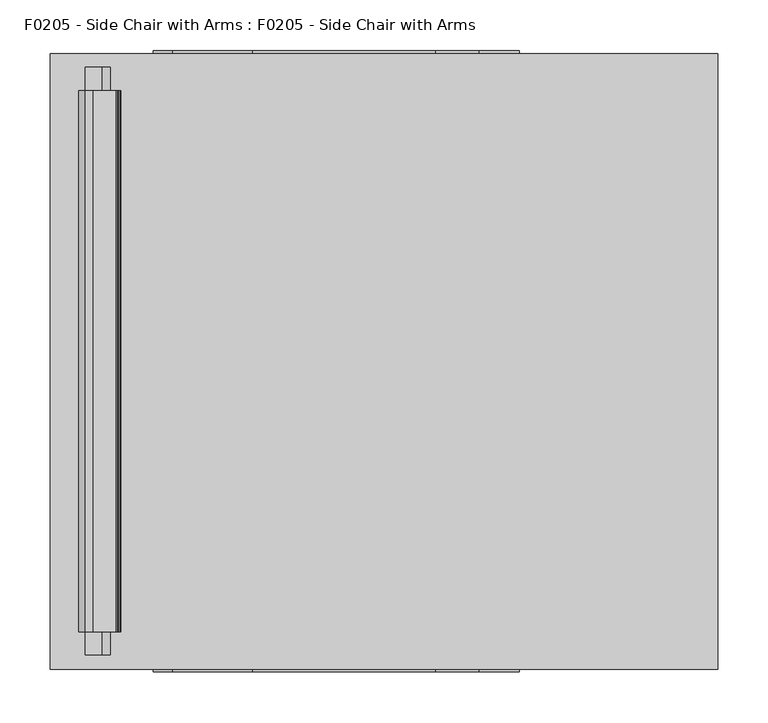
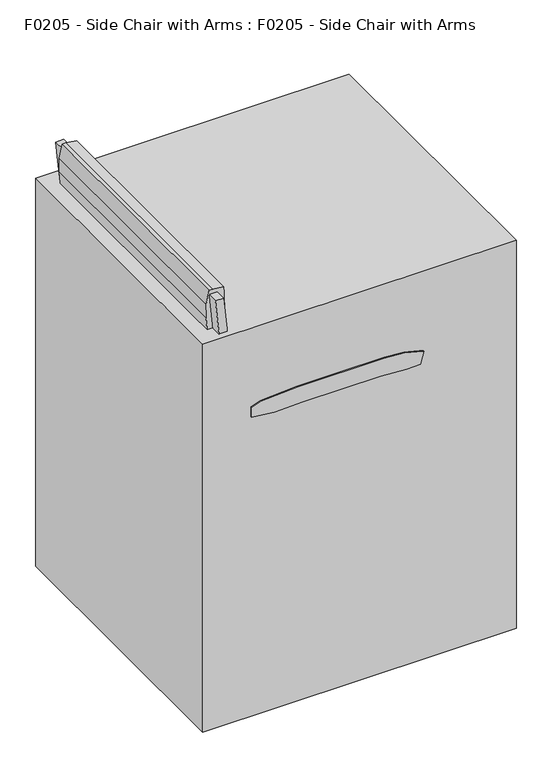
"""IFC4 building model written with IfcOpenShell, lengths in millimetres: proxy geometry, F0205 - Side Chair with Arms : F0205 - Side Chair with Arms."""

import ifcopenshell
import ifcopenshell.guid

model = None  # the IFC model being written
_history = None  # IfcOwnerHistory: only IFC2X3 demands one
_inside = {}  # id of a spatial element -> (the spatial element, [elements in it])
_under = {}  # id of a project, library or spatial element -> (it, [spatial elements below it])
_declared = {}  # id of a project -> (the project, [libraries it declares])
_typed = {}  # id of a type object -> (the type object, [elements of that type])
_made_of = {}  # id of a material, layer set ... -> (it, [elements and type objects made of it])


def new_model(schema):
    """Start an empty IFC model of exactly this schema.

    Asked for "IFC4X3", IfcOpenShell would pick the latest addendum, in which some entities
    have other attributes; the version numbers below select the first issue.
    IFC2X3 requires an IfcOwnerHistory on every rooted entity: one is made here for all.
    """
    global model, _history
    if schema == "IFC4X3":
        model = ifcopenshell.file(schema_version=(4, 3, 0, 0))
    else:
        model = ifcopenshell.file(schema=schema)
    _inside.clear()
    _under.clear()
    _declared.clear()
    _typed.clear()
    _made_of.clear()
    _history = None
    if model.schema == "IFC2X3":
        org = make("IfcOrganization", Name="unknown")
        user = make(
            "IfcPersonAndOrganization",
            ThePerson=make("IfcPerson", FamilyName="unknown"),
            TheOrganization=org,
        )
        app = make(
            "IfcApplication",
            ApplicationDeveloper=org,
            Version="unknown",
            ApplicationFullName="unknown",
            ApplicationIdentifier="unknown",
        )
        _history = make(
            "IfcOwnerHistory",
            OwningUser=user,
            OwningApplication=app,
            ChangeAction="ADDED",
            CreationDate=0,
        )
    return model


def make(cls, **values):
    """One entity of the class cls with the attributes given. An attribute that is None is left unset."""
    return model.create_entity(
        cls, **{name: value for name, value in values.items() if value is not None}
    )


def rooted(cls, **values):
    """An entity with a GlobalId (a new one), such as an element, a storey or a relation."""
    return make(cls, GlobalId=ifcopenshell.guid.new(), OwnerHistory=_history, **values)


def si_unit(unit_type, name, prefix=None):
    """IfcSIUnit, for example si_unit("LENGTHUNIT", "METRE", prefix="MILLI")."""
    return make("IfcSIUnit", UnitType=unit_type, Prefix=prefix, Name=name)


def assignment(units):
    """IfcUnitAssignment: the units of a project."""
    return None if units is None else make("IfcUnitAssignment", Units=units)


def point(xyz):
    """IfcCartesianPoint."""
    return None if xyz is None else make("IfcCartesianPoint", Coordinates=xyz)


def direction(xyz):
    """IfcDirection."""
    return None if xyz is None else make("IfcDirection", DirectionRatios=xyz)


def frame(location, z_axis=None, x_axis=None):
    """IfcAxis2Placement3D, a coordinate frame: its origin and axes. An axis left out is left unset."""
    return make(
        "IfcAxis2Placement3D",
        Location=point(location),
        Axis=direction(z_axis),
        RefDirection=direction(x_axis),
    )


def origin():
    """The frame at (0, 0, 0) with its axes left unset."""
    return frame((0.0, 0.0, 0.0))


def origin_with_axes():
    """The frame at (0, 0, 0) with the z axis (0, 0, 1) and the x axis (1, 0, 0) written out."""
    return frame((0.0, 0.0, 0.0), z_axis=(0.0, 0.0, 1.0), x_axis=(1.0, 0.0, 0.0))


def place(relative_to, where):
    """IfcLocalPlacement: puts the frame where relative to a parent placement (None: the world)."""
    return make(
        "IfcLocalPlacement", PlacementRelTo=relative_to, RelativePlacement=where
    )


def context(
    kind, dimensions, precision=None, world=None, true_north=None, identifier=None
):
    """IfcGeometricRepresentationContext, for example the 3D "Model" context."""
    return make(
        "IfcGeometricRepresentationContext",
        ContextIdentifier=identifier,
        ContextType=kind,
        CoordinateSpaceDimension=dimensions,
        Precision=precision,
        WorldCoordinateSystem=world,
        TrueNorth=true_north,
    )


def project(units=None, contexts=None):
    """IfcProject with its units and contexts."""
    return rooted(
        "IfcProject",
        Name="project",
        RepresentationContexts=contexts,
        UnitsInContext=assignment(units),
    )


def spatial(cls, under=None, at=None, **own):
    """A site, building, storey or space (cls), placed at a placement, below another one or the project."""
    s = rooted(cls, ObjectPlacement=at, **own)
    if under is not None:
        _under.setdefault(under.id(), (under, []))[1].append(s)
    return s


def polyline(points):
    """IfcPolyline through the points."""
    return make("IfcPolyline", Points=[point(p) for p in points])


def outline(outer, holes=None, kind="AREA"):
    """IfcArbitraryClosedProfileDef: a profile drawn as a closed curve; with holes, ...WithVoids."""
    if holes is None:
        return make("IfcArbitraryClosedProfileDef", ProfileType=kind, OuterCurve=outer)
    return make(
        "IfcArbitraryProfileDefWithVoids",
        ProfileType=kind,
        OuterCurve=outer,
        InnerCurves=holes,
    )


def extrude(swept, where, along, depth):
    """IfcExtrudedAreaSolid: the profile swept, set in the frame where, extruded along a direction by depth."""
    return make(
        "IfcExtrudedAreaSolid",
        SweptArea=swept,
        Position=where,
        ExtrudedDirection=direction(along),
        Depth=depth,
    )


def shape(context_of_items, identifier, shape_type, items):
    """IfcShapeRepresentation: the items that make up one representation, for example the "Body"."""
    return make(
        "IfcShapeRepresentation",
        ContextOfItems=context_of_items,
        RepresentationIdentifier=identifier,
        RepresentationType=shape_type,
        Items=items,
    )


def source(mapping_origin, context_of_items, identifier, shape_type, items):
    """IfcRepresentationMap: a shape defined once, which mapped items show again and again."""
    return make(
        "IfcRepresentationMap",
        MappingOrigin=mapping_origin,
        MappedRepresentation=shape(context_of_items, identifier, shape_type, items),
    )


def transform(
    local_origin,
    x_axis=None,
    y_axis=None,
    z_axis=None,
    scale=None,
    scale2=None,
    scale3=None,
    uniform=True,
):
    """IfcCartesianTransformationOperator3D, or its non-uniform kind. x_axis, y_axis, z_axis: its Axis1, 2, 3."""
    if uniform:
        return make(
            "IfcCartesianTransformationOperator3D",
            Axis1=direction(x_axis),
            Axis2=direction(y_axis),
            LocalOrigin=point(local_origin),
            Scale=scale,
            Axis3=direction(z_axis),
        )
    return make(
        "IfcCartesianTransformationOperator3DnonUniform",
        Axis1=direction(x_axis),
        Axis2=direction(y_axis),
        LocalOrigin=point(local_origin),
        Scale=scale,
        Axis3=direction(z_axis),
        Scale2=scale2,
        Scale3=scale3,
    )


def mapped(mapping_source, mapping_target):
    """IfcMappedItem: shows the shape of a source again, moved by a transform."""
    return make(
        "IfcMappedItem", MappingSource=mapping_source, MappingTarget=mapping_target
    )


def made_of(thing, what):
    """Note that an element or type object is made of a material, layer set ...; save() writes the relation."""
    if what is not None:
        _made_of.setdefault(what.id(), (what, []))[1].append(thing)
    return thing


def element(
    cls,
    number,
    at=None,
    inside=None,
    cuts=None,
    type_object=None,
    material=None,
    context=None,
    identifier="Body",
    shape_type=None,
    held_by="IfcProductDefinitionShape",
    body=None,
    shapes=None,
    **own,
):
    """One element of the class cls, such as IfcWall. Its Tag is "e" and its number.

    at: its placement. inside: the storey or other place that contains it. cuts: it is an
    opening in that element (IfcRelVoidsElement). A single representation is given by context,
    identifier, shape_type and body (its items); several are given by shapes. held_by: the class
    of the entity that holds the representations. save() writes the other relations.
    """
    e = rooted(cls, Tag="e%d" % number, ObjectPlacement=at, **own)
    if body is not None:
        shapes = [shape(context, identifier, shape_type, body)]
    if shapes is not None:
        e.Representation = make(held_by, Representations=shapes)
    if inside is not None:
        _inside.setdefault(inside.id(), (inside, []))[1].append(e)
    if cuts is not None:
        rooted(
            "IfcRelVoidsElement", RelatingBuildingElement=cuts, RelatedOpeningElement=e
        )
    if type_object is not None:
        _typed.setdefault(type_object.id(), (type_object, []))[1].append(e)
    return made_of(e, material)


def aggregate(whole, parts):
    """IfcRelAggregates: a whole, such as a stair, and the parts it consists of."""
    return rooted("IfcRelAggregates", RelatingObject=whole, RelatedObjects=parts)


def save(model, path):
    """Write the relations noted so far, then the file.

    IfcRelAggregates (storeys below a building ...), IfcRelContainedInSpatialStructure (elements
    in a storey), IfcRelDefinesByType, IfcRelAssociatesMaterial and IfcRelDeclares: one each for
    every whole, place, type object, material and project.
    """
    for whole, parts in _under.values():
        aggregate(whole, parts)
    for where, things in _inside.values():
        rooted(
            "IfcRelContainedInSpatialStructure",
            RelatedElements=things,
            RelatingStructure=where,
        )
    for kind, things in _typed.values():
        rooted("IfcRelDefinesByType", RelatedObjects=things, RelatingType=kind)
    for what, things in _made_of.values():
        rooted("IfcRelAssociatesMaterial", RelatedObjects=things, RelatingMaterial=what)
    for by, libraries in _declared.values():
        rooted("IfcRelDeclares", RelatingContext=by, RelatedDefinitions=libraries)
    model.write(path)


def f0205_side_chair_with_arms_f0205_side_chair_with_arms_598bf5c1(model_context):
    return source(origin(), model_context, "Body", "SweptSolid", [
        extrude(outline(polyline([(949.5558695, -288.1891828), (949.0276678, -295.7428189), (920.9464532, -302.0388283), (890.9596762, -302.364601), (766.4444592, -291.4709311), (712.0444312, -282.2922915), (699.4048634, -275.0755148), (701.6800869, -249.0695909), (734.5347731, -247.5019251), (744.2301544, -248.5209507), (775.1826091, -252.8120869), (831.1136295, -257.7054171), (872.5802588, -261.3332771), (887.0899422, -262.6027099), (935.3234911, -264.152458), (946.525946, -265.1325458), (949.5558695, -288.1891828)])), frame((0.0, -267.8488342, 0.0), z_axis=(0.0, 1.0, 0.0), x_axis=(0.0, 0.0, 1.0)), (0.0, 0.0, 1.0), 536.2041409),
        extrude(outline(polyline([(-256.4009052, 523.5214117), (-241.6696752, 524.0358376), (0.2532363, 511.5153378), (242.1729901, 524.0426254), (256.8914817, 523.5286444), (268.3553067, 472.7447876), (248.2006555, 466.9655344), (0.2531025, 454.1861401), (-247.7015659, 466.8926254), (-267.8488342, 472.7447876), (-256.4009052, 523.5214117)])), frame((-276.0175852, 0.0, 0.0), z_axis=(1.0, 0.0, 0.0), x_axis=(0.0, 1.0, 0.0)), (0.0, 0.0, 1.0), 448.6997704),
        extrude(outline(polyline([(688.7736743, -228.6), (667.1445431, -228.6), (661.9341602, -181.3714246), (664.006805, -120.3965081), (664.006805, 42.1384065), (660.8978378, 96.9044584), (660.8978378, 126.6899316), (687.4154537, 134.0660802), (697.5043243, 94.4420938), (700.8875965, 51.2519248), (700.8875965, -129.7992697), (695.7892437, -209.3248816), (688.7736743, -228.6)])), frame((0.0, -307.5947608, 0.0), z_axis=(0.0, 1.0, 0.0), x_axis=(0.0, 0.0, 1.0)), (0.0, 0.0, 1.0), 60.4113562),
        extrude(outline(polyline([(688.7736743, -228.6), (667.1445431, -228.6), (661.9341602, -181.3714246), (664.006805, -120.3965081), (664.006805, 42.1384065), (667.1445431, -13.1344595), (667.1445431, 128.4275172), (687.4154537, 134.0660802), (697.5043243, 94.4420938), (700.8875965, 51.2519248), (700.8875965, -129.7992697), (695.7892437, -209.3248816), (688.7736743, -228.6)])), frame((0.0, 248.2080384, 0.0), z_axis=(0.0, 1.0, 0.0), x_axis=(0.0, 0.0, 1.0)), (0.0, 0.0, 1.0), 59.893195),
        extrude(outline(polyline([(504.8449262, 147.1860068), (504.8449262, -258.5366203), (479.5415809, -260.4830005), (479.5415809, 149.3997627), (504.8449262, 147.1860068)])), frame((0.0, -290.8917348, 0.0), z_axis=(0.0, 1.0, 0.0), x_axis=(0.0, 0.0, 1.0)), (0.0, 0.0, 1.0), 25.4),
        extrude(outline(polyline([(504.8449262, 147.1860068), (504.8449262, -258.5366203), (479.5415809, -260.4830005), (479.5415809, 149.3997627), (504.8449262, 147.1860068)])), frame((0.0, 264.3929274, 0.0), z_axis=(0.0, 1.0, 0.0), x_axis=(0.0, 0.0, 1.0)), (0.0, 0.0, 1.0), 25.4),
        extrude(outline(polyline([(0.0, -297.370228), (642.1831371, -247.9723105), (642.1831371, 101.2776895), (617.1504769, 126.3103497), (505.0230984, 147.1704188), (0.0, 191.3542147), (0.0, 215.7503897), (505.0203406, 172.091969), (627.5762276, 149.2917903), (667.1445431, 107.5467505), (667.1445431, -250.1263819), (940.2581485, -278.8317785), (940.2581485, -295.7126518), (642.1831371, -266.7616436), (0.0, -322.770228), (0.0, -297.370228)])), frame((0.0, -290.8917348, 0.0), z_axis=(0.0, 1.0, 0.0), x_axis=(0.0, 0.0, 1.0)), (0.0, 0.0, 1.0), 26.9964161),
        extrude(outline(polyline([(0.0, -297.370228), (642.1831371, -247.9723105), (642.1831371, 101.2776895), (617.1504769, 126.3103497), (505.0230984, 147.1704188), (0.0, 191.3542147), (0.0, 215.7503897), (505.0203406, 172.091969), (627.5762276, 149.2917903), (667.1445431, 107.5467505), (667.1445431, -250.1263819), (940.2581485, -278.8317785), (940.2581485, -295.7126518), (642.1831371, -266.7616436), (0.0, -322.770228), (0.0, -297.370228)])), frame((0.0, 264.3929274, 0.0), z_axis=(0.0, 1.0, 0.0), x_axis=(0.0, 0.0, 1.0)), (0.0, 0.0, 1.0), 26.9964161),
        extrude(outline(polyline([(330.2, 304.8), (330.2, -304.8), (-330.2, -304.8), (-330.2, 304.8), (330.2, 304.8)])), origin_with_axes(), (0.0, 0.0, 1.0), 863.6),
    ])


if __name__ == "__main__":
    model = new_model("IFC4")
    model_context = context("Model", 3, world=origin())
    ifc_project = project(units=[si_unit("LENGTHUNIT", "METRE", prefix="MILLI")], contexts=[model_context])
    site = spatial("IfcSite", under=ifc_project)
    building = spatial("IfcBuilding", under=site)
    placement = place(None, origin())
    f0205_side_chair_with_arms_f0205_side_chair_with_arms_shape = f0205_side_chair_with_arms_f0205_side_chair_with_arms_598bf5c1(model_context)
    element("IfcBuildingElementProxy", 1, Name="F0205 - Side Chair with Arms : F0205 - Side Chair with Arms", ObjectType="F0205 - Side Chair with Arms : F0205 - Side Chair with Arms", at=placement, inside=building, context=model_context, shape_type="MappedRepresentation", body=[
        mapped(f0205_side_chair_with_arms_f0205_side_chair_with_arms_shape, transform((0.0, 0.0, 0.0), x_axis=(1.0, 0.0, 0.0), y_axis=(0.0, 1.0, 0.0), z_axis=(0.0, 0.0, 1.0))),
    ])
    save(model, "model.ifc")

# Revit data of these elements
# Project information
#   Sheets - Total = "6"
#   Project Issue Date = "Issue Date"
#   Project Status = "Project Status"
#   Client Name = "Owner"
#   Project Address = "Enter address here"
#   Project Name = "Project Name"
#   Project Number = "Project Number"
#   Publication Date = "30-Jan-15"
# Type "F0205 - Side Chair with Arms : F0205 - Side Chair with Arms"
#   Watts2 = "0"
#   Watts1 = "0"
#   Unit_Issue = "EA"
#   UTIL_6_Misc = "-"
#   UTIL_5_NonMedGas = "-"
#   UTIL_4_MiscGas = "-"
#   UTIL_3_MedGas = "-"
#   UTIL_2_Elec = "-"
#   UTIL_1_WaterDrain = "-"
#   Nomenclature = "Chair, Side With Arms"
#   NSN = "7110"
#   Location [instance default] = ""
#   JSN = "F0205"
#   Fund_Source_VA = "-"
#   Fund_Source_Navy = "-"
#   Fund_Source_Army = "-"
#   Fund_Source_AF = "-"
#   ELEC_Volts2 = "0"
#   ELEC_Volts1 = "0"
#   ELEC_Phase2 = "0"
#   ELEC_Phase1 = "0"
#   ELEC_HertzSwitch = "0"
#   ELEC_HertzDependent = "0"
#   ELEC_Hertz = "0"
#   ELEC_Amps2 = "0"
#   ELEC_Amps1 = "0"
#   DetailDescription = "Upholstered side chair, 32\" high X 21\" wide X 23\" deep with arms, padded seats and padded backs. Seat height is a minimum of 17\".  Available with or without sled base."
#   CAT_VA = "C"
#   CAT_Navy = "C"
#   CAT_IHS = "-"
#   CAT_Army = "C"
#   CAT_AF = "C"
#   BTUperhour = "0"
#   Weight_IP = 42
#   DIM_Width_IP = 2' - 0"
#   DIM_Height_IP = 2' - 10"
#   DIM_Depth_IP = 2' - 2"
#   Assembly Code = ""
# Element 1 (IfcBuildingElementProxy, "F0205 - Side Chair with Arms : F0205 - Side Chair with Arms")
#   Location = "OPTM1"
#   Materials on its faces: "ChairFabric", "EquipSpace"
# Materials
#   "ChairFabric": class "Unassigned", colour RGB 188 173 117, transparency 0
#   "EquipSpace": class "Unassigned", colour RGB 221 217 195, transparency 0.5
